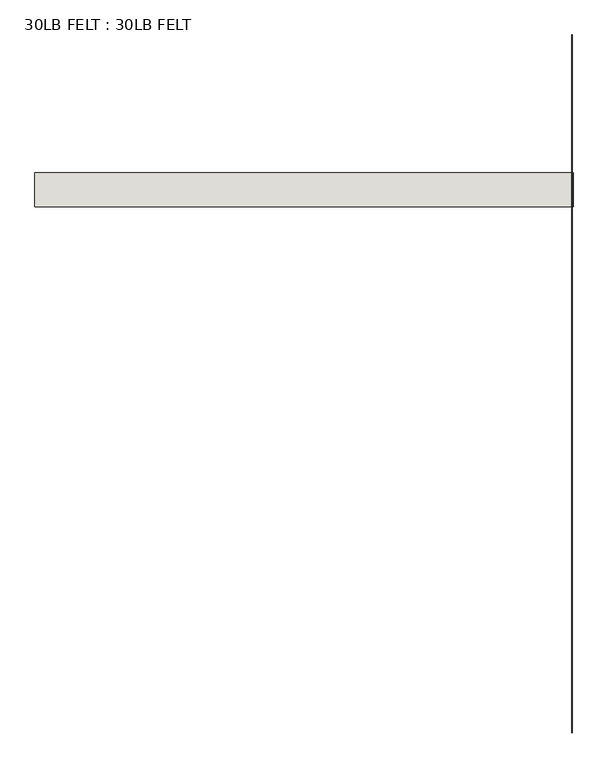
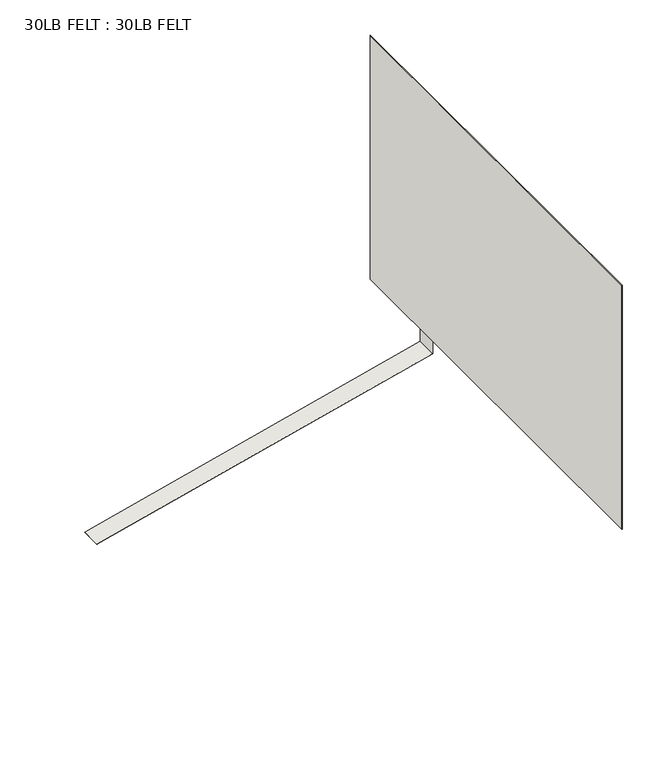
"""IFC4 building model written with IfcOpenShell, lengths in millimetres: wall geometry, 30LB FELT : 30LB FELT."""

from ifc_helpers import new_model, si_unit, frame, origin, place, context, project, spatial, polyline, outline, extrude, source, transform, mapped, element, save


def wall_30lb_felt_30lb_felt_add5ed2b(model_context):
    return source(origin(), model_context, "Body", "SweptSolid", [
        extrude(outline(polyline([(3129.9096218, 19596.0857949), (3129.9096218, 19594.4982949), (2950.7936288, 19594.4982949), (2399.4695676, 17389.20205), (2397.9292228, 17389.5861011), (2949.5541463, 19596.0857949), (3129.9096218, 19596.0857949)])), frame((0.0, -1256.0384634, 0.0), z_axis=(0.0, 1.0, 0.0), x_axis=(0.0, 0.0, 1.0)), (0.0, 0.0, 1.0), 139.7),
        extrude(outline(polyline([(4732.6932155, 19590.1475817), (3041.7352617, 19590.1475817), (3041.7352617, 19591.7350817), (4735.8682155, 19591.7350817), (4732.6932155, 19590.1475817)])), frame((0.0, -3415.0384634, 0.0), z_axis=(0.0, 1.0, 0.0), x_axis=(0.0, 0.0, 1.0)), (0.0, 0.0, 1.0), 2862.7206389),
    ])


if __name__ == "__main__":
    model = new_model("IFC4")
    model_context = context("Model", 3, world=origin())
    ifc_project = project(units=[si_unit("LENGTHUNIT", "METRE", prefix="MILLI")], contexts=[model_context])
    site = spatial("IfcSite", under=ifc_project)
    building = spatial("IfcBuilding", under=site)
    placement = place(None, origin())
    wall_30lb_felt_30lb_felt_shape = wall_30lb_felt_30lb_felt_add5ed2b(model_context)
    element("IfcWall", 1, ObjectType="30LB FELT : 30LB FELT", at=placement, inside=building, context=model_context, shape_type="MappedRepresentation", body=[
        mapped(wall_30lb_felt_30lb_felt_shape, transform((0.0, 0.0, 0.0), x_axis=(1.0, 0.0, 0.0), y_axis=(0.0, 1.0, 0.0), z_axis=(0.0, 0.0, 1.0))),
    ])
    save(model, "model.ifc")

# Revit data of these elements
# Element 1 (IfcWall, "30LB FELT : 30LB FELT")
#   Materials on its faces: "30LB FELT", "WRB"
# Materials
#   "30LB FELT": class "Generic", colour RGB 66 158 52, transparency 0, Cost = 0
#   "WRB": class "Generic", colour RGB 66 158 52, transparency 0, Cost = 0
